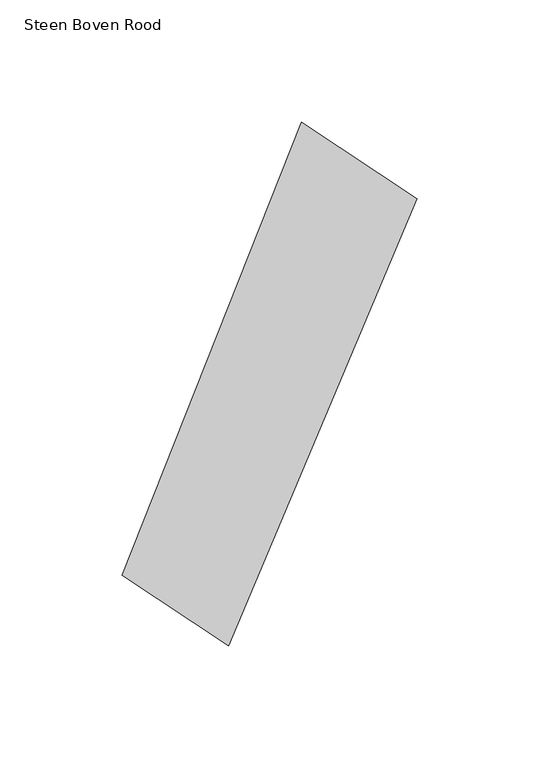
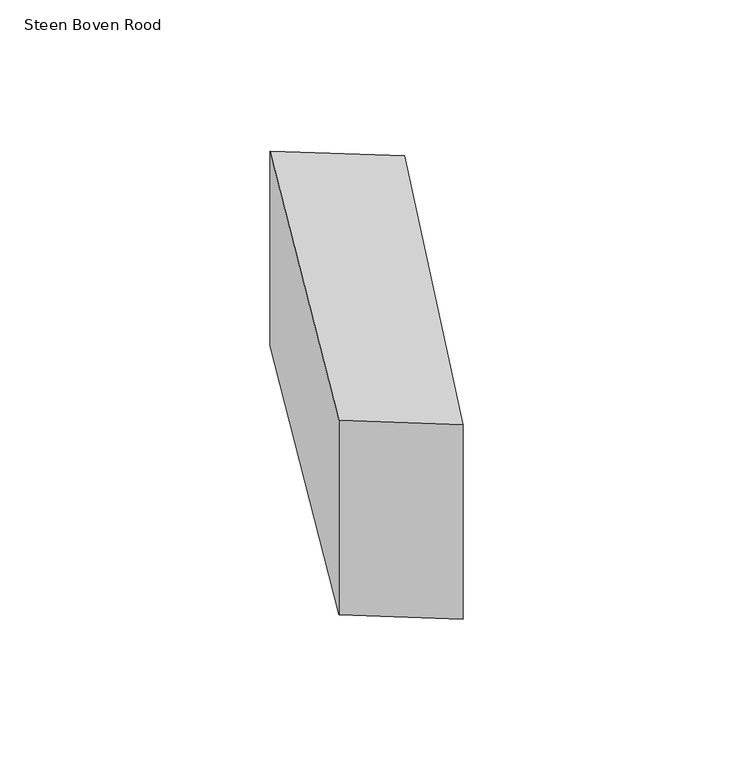
"""IFC4 building model written with IfcOpenShell, lengths in millimetres: proxy geometry, 00_GMA_steen_versie_4 : Steen Boven Rood."""

from ifc_helpers import new_model, si_unit, origin, origin_with_axes, place, context, project, spatial, polyline, outline, extrude, source, transform, mapped, element, save


def steen_boven_rood_37eec749(model_context):
    return source(origin(), model_context, "Body", "SweptSolid", [
        extrude(outline(polyline([(140.9146831, 165.1376864), (63.7989312, -17.8120628), (20.1809605, 11.094439), (93.6898266, 196.4573931), (140.9146831, 165.1376864)])), origin_with_axes(), (0.0, 0.0, 1.0), 100.0),
    ])


if __name__ == "__main__":
    model = new_model("IFC4")
    model_context = context("Model", 3, world=origin())
    ifc_project = project(units=[si_unit("LENGTHUNIT", "METRE", prefix="MILLI")], contexts=[model_context])
    site = spatial("IfcSite", under=ifc_project)
    building = spatial("IfcBuilding", under=site)
    placement = place(None, origin())
    steen_boven_rood_shape = steen_boven_rood_37eec749(model_context)
    element("IfcBuildingElementProxy", 1, Name="00_GMA_steen_versie_4 : Steen Boven Rood", ObjectType="00_GMA_steen_versie_4 : Steen Boven Rood", at=placement, inside=building, context=model_context, shape_type="MappedRepresentation", body=[
        mapped(steen_boven_rood_shape, transform((0.0, 0.0, 0.0), x_axis=(1.0, 0.0, 0.0), y_axis=(0.0, 1.0, 0.0), z_axis=(0.0, 0.0, 1.0))),
    ])
    save(model, "model.ifc")

# Revit data of these elements
# Type "00_GMA_steen_versie_4 : Steen Boven Rood"
#   StootVoegHalfBoven [instance default] = 5 mm
#   StootVoegHalf [instance default] = 5 mm
#   StootVoegBreedteOnder = 10 mm
#   StootVoegBreedteBoven = 10 mm
#   Steendikte = 100 mm
#   LintVoegOnderHalf = 5 mm
#   LintVoegOnder = 10 mm
#   LintVoegBovenHalf = 0 mm
#   LintVoegBoven = 0 mm
#   materiaal = 21_steen_rood
#   MateriaalVoeg = none
#   Default Elevation = 0
# Element 1 (IfcBuildingElementProxy, "00_GMA_steen_versie_4 : Steen Boven Rood")
#   Materials on its faces: "21_steen_rood"
# Materials
#   "21_steen_rood": class "Unassigned", colour RGB 213 111 43, transparency 0, Cost = 0
